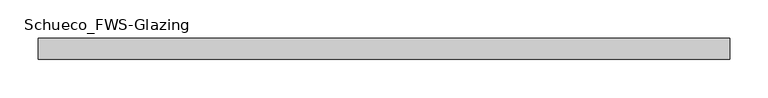
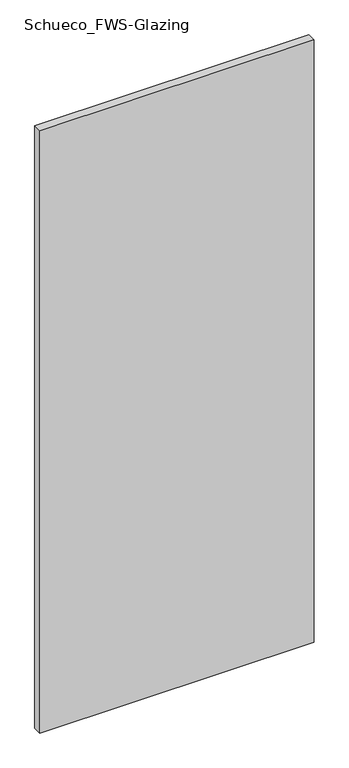
"""IFC4 building model written with IfcOpenShell, lengths in millimetres: plate geometry, Schueco_FWS-Glazing : HI_28mm_DoubGlz."""

from ifc_helpers import new_model, si_unit, origin, origin_with_axes, place, context, project, spatial, polyline, outline, extrude, source, transform, mapped, element, save


def schueco_fws_glazing_2d8adcb3(model_context):
    return source(origin(), model_context, "Body", "SweptSolid", [
        extrude(outline(polyline([(454.0, -28.0), (-454.0, -28.0), (-454.0, 0.0), (454.0, 0.0), (454.0, -28.0)])), origin_with_axes(), (0.0, 0.0, 1.0), 2108.0),
    ])


if __name__ == "__main__":
    model = new_model("IFC4")
    model_context = context("Model", 3, world=origin())
    ifc_project = project(units=[si_unit("LENGTHUNIT", "METRE", prefix="MILLI")], contexts=[model_context])
    site = spatial("IfcSite", under=ifc_project)
    building = spatial("IfcBuilding", under=site)
    placement = place(None, origin())
    schueco_fws_glazing_shape = schueco_fws_glazing_2d8adcb3(model_context)
    element("IfcPlate", 1, ObjectType="Schueco_FWS-Glazing : HI_28mm_DoubGlz", at=placement, inside=building, context=model_context, shape_type="MappedRepresentation", body=[
        mapped(schueco_fws_glazing_shape, transform((0.0, 0.0, 0.0), x_axis=(1.0, 0.0, 0.0), y_axis=(0.0, 1.0, 0.0), z_axis=(0.0, 0.0, 1.0))),
    ])
    save(model, "model.ifc")

# Revit data of these elements
# Type "Schueco_FWS-Glazing : HI_28mm_DoubGlz"
#   Model = "Double glazing 28mm"
#   Manufacturer = "Schueco International KG"
#   Analytic Construction = "<Keine Auswahl>"
#   Glazing thickness = 28 mm
#   FWS SI insert unit = no
#   FWS HI insert unit = yes
#   Glass = Glass
# Element 1 (IfcPlate, "Schueco_FWS-Glazing : HI_28mm_DoubGlz")
#   Materials on its faces: "Glass"
# Materials
#   "Glass": class "Glass", colour RGB 128 128 255, transparency 0.75, Description = "Soda Lime Glass", Cost = 0
